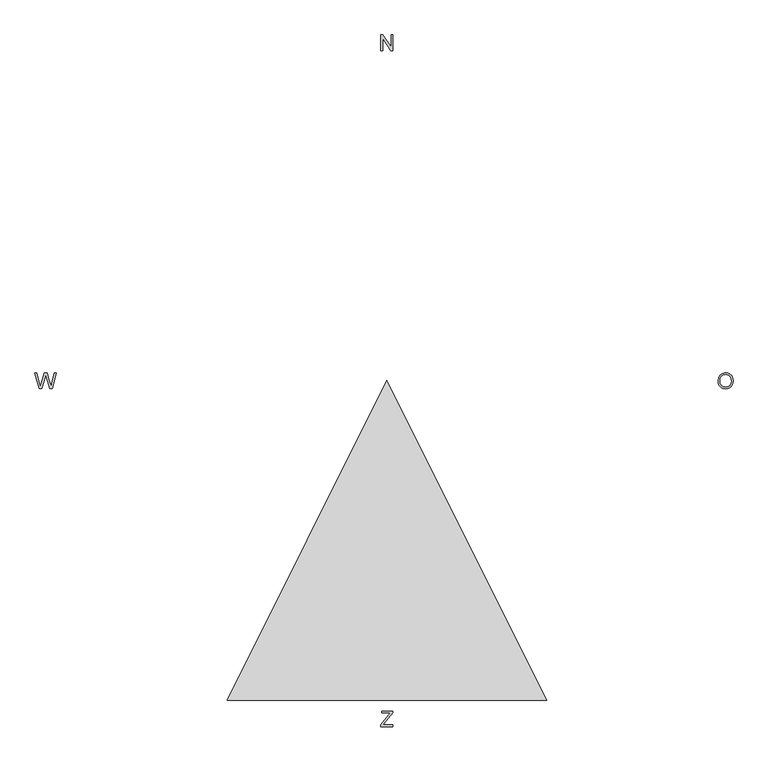
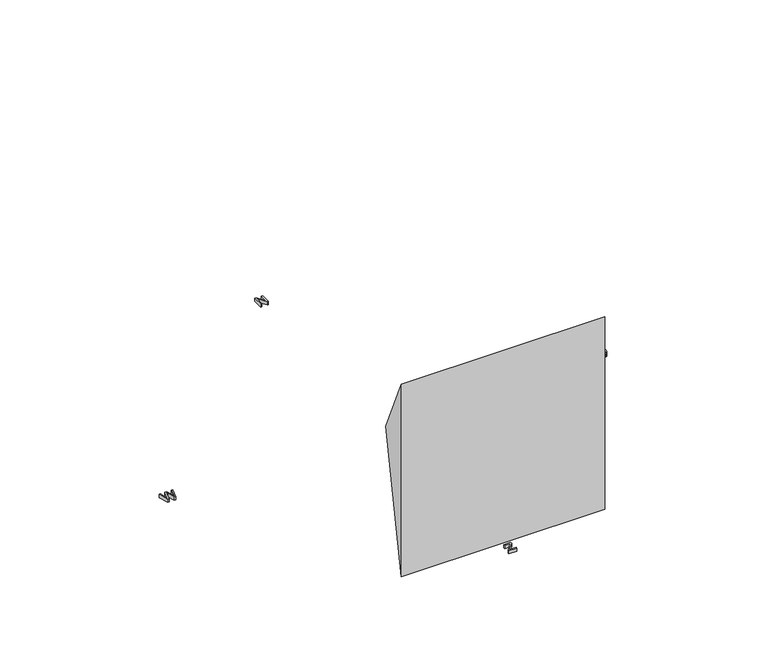
"""IFC4 building model written with IfcOpenShell, lengths in millimetres: geographic element geometry, 00.40_SI_BIMbasisInfra_Referentiepunt : coördinatie punt."""

from ifc_helpers import new_model, si_unit, origin, origin_with_axes, place, context, project, spatial, polyline, outline, extrude, faceted_brep, source, transform, mapped, element, save


def geographic_element_aab1c94c(model_context):
    return source(origin(), model_context, "Body", "SolidModel", [
        extrude(outline(polyline([(3109.2307692, -3.1009615), (3114.1526442, 29.5582933), (3128.9182692, 54.2668269), (3151.4633413, 69.8167067), (3179.7235577, 75.0), (3199.0955529, 72.5661058), (3216.4663462, 65.2644231), (3230.8894231, 53.608774), (3241.4182692, 38.1129808), (3247.8545673, 19.5252404), (3250.0, -1.40625), (3247.741887, -22.6171875), (3240.9675481, -41.4663462), (3230.0510817, -56.9891827), (3215.3665865, -68.2211538), (3198.1445313, -75.0360577), (3179.6153846, -77.3076923), (3159.9459135, -74.7971755), (3142.4759615, -67.265625), (3128.0889423, -55.3936298), (3117.6682692, -39.8617788), (3111.3401442, -21.9906851), (3109.2307692, -3.1009615)]), holes=[polyline([(3127.6923077, -3.28125), (3131.3837139, -26.3852163), (3142.4579327, -43.9903846), (3159.1030649, -55.1322115), (3179.5072115, -58.8461538), (3200.2088341, -55.0961538), (3216.8810096, -43.8461538), (3227.8740986, -25.7001202), (3231.5384615, -1.2620192), (3229.9699519, 15.0811298), (3225.2644231, 29.2067308), (3217.5435697, 40.7587139), (3206.9290865, 49.3810096), (3194.1240986, 54.7490986), (3179.8317308, 56.5384615), (3159.9729567, 53.0904447), (3143.0889423, 42.7463942), (3131.5414663, 24.3434495), (3127.6923077, -3.28125)])]), origin_with_axes(), (0.0, 0.0, 1.0), 50.0),
        extrude(outline(polyline([(-3262.8004808, -75.0), (-3303.0769231, 72.6923077), (-3284.0384615, 72.6923077), (-3260.6730769, -24.375), (-3253.4615385, -54.3389423), (-3245.7451923, -27.8365385), (-3216.4663462, 72.6923077), (-3189.0264423, 72.6923077), (-3167.7524038, -0.1802885), (-3151.9230769, -54.3389423), (-3144.9278846, -25.2403846), (-3121.3822115, 72.6923077), (-3102.3076923, 72.6923077), (-3142.5480769, -75.0), (-3162.3076923, -75.0), (-3197.7524038, 38.9423077), (-3202.6923077, 54.84375), (-3208.2451923, 35.6971154), (-3240.5168269, -75.0), (-3262.8004808, -75.0)])), origin_with_axes(), (0.0, 0.0, 1.0), 50.0),
        extrude(outline(polyline([(-57.6923077, -3250.0), (-57.6923077, -3230.8533654), (17.8125, -3138.3293269), (32.1634615, -3120.7692308), (-48.4615385, -3120.7692308), (-48.4615385, -3102.3076923), (55.3846154, -3102.3076923), (55.3846154, -3120.7692308), (-27.2596154, -3222.0192308), (-35.0480769, -3231.5384615), (57.6923077, -3231.5384615), (57.6923077, -3250.0), (-57.6923077, -3250.0)])), origin_with_axes(), (0.0, 0.0, 1.0), 50.0),
        extrude(outline(polyline([(-57.6923077, 3100.0), (-57.6923077, 3247.6923077), (-37.9326923, 3247.6923077), (39.2307692, 3130.6850962), (39.2307692, 3247.6923077), (57.6923077, 3247.6923077), (57.6923077, 3100.0), (37.9326923, 3100.0), (-39.2307692, 3217.0432692), (-39.2307692, 3100.0), (-57.6923077, 3100.0)])), origin_with_axes(), (0.0, 0.0, 1.0), 50.0),
        faceted_brep([(1500.0, -3000.0, 0.0), (0.0, 0.0, 0.0), (1500.0, -3000.0, 3000.0), (-1500.0, -3000.0, 0.0), (-1500.0, -3000.0, 3000.0)], [[[0, 1, 2]], [[3, 0, 2, 4]], [[4, 2, 1]], [[1, 3, 4]], [[3, 1, 0]]]),
    ])


if __name__ == "__main__":
    model = new_model("IFC4")
    model_context = context("Model", 3, world=origin())
    ifc_project = project(units=[si_unit("LENGTHUNIT", "METRE", prefix="MILLI")], contexts=[model_context])
    site = spatial("IfcSite", under=ifc_project)
    building = spatial("IfcBuilding", under=site)
    placement = place(None, origin())
    geographic_element_shape = geographic_element_aab1c94c(model_context)
    element("IfcGeographicElement", 1, ObjectType="00.40_SI_BIMbasisInfra_Referentiepunt : coördinatie punt", at=placement, inside=building, context=model_context, shape_type="MappedRepresentation", body=[
        mapped(geographic_element_shape, transform((0.0, 0.0, 0.0), x_axis=(1.0, 0.0, 0.0), y_axis=(0.0, 1.0, 0.0), z_axis=(0.0, 0.0, 1.0))),
    ])
    save(model, "model.ifc")

# Revit data of these elements
# Type "00.40_SI_BIMbasisInfra_Referentiepunt : coördinatie punt"
#   Type Comments = ""
#   Description = ""
#   Assembly Code = "00.40"
#   Default Elevation = 0
# Element 1 (IfcGeographicElement, "00.40_SI_BIMbasisInfra_Referentiepunt : coördinatie punt")
#   Materials on its faces: "0-punt-letters", "0-punt"
# Materials
#   "0-punt-letters": class "Unassigned", colour RGB 160 205 219, transparency 0.1, Cost = 0
#   "0-punt": class "Unassigned", colour RGB 73 146 116, transparency 0, Cost = 0
